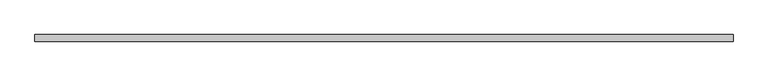
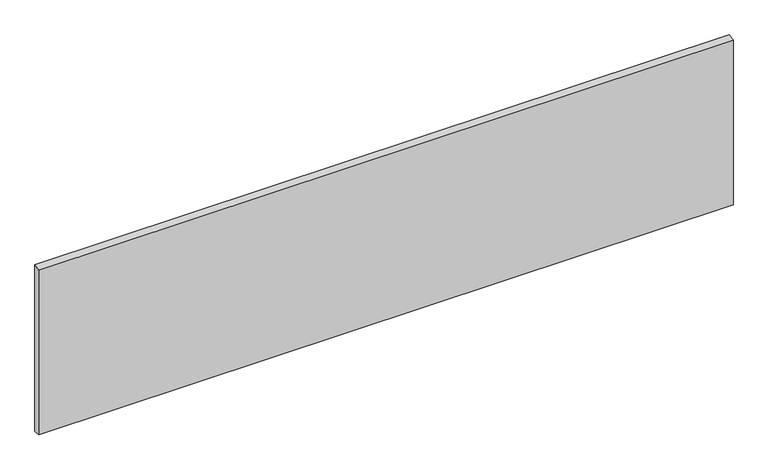
"""IFC4 building model written with IfcOpenShell, lengths in millimetres: proxy geometry, Plywood018 952 : Plywood018 952."""

from ifc_helpers import new_model, si_unit, frame, origin, place, context, project, spatial, polyline, outline, extrude, source, transform, mapped, element, save


def generic_models_6d488722(model_context):
    return source(origin(), model_context, "Body", "SweptSolid", [
        extrude(outline(polyline([(10417.7250834, 42906.696), (10417.7250834, 43408.1095103), (10436.7750834, 43412.8720103), (10436.7750834, 42906.696), (10417.7250834, 42906.696)])), frame((3694.2883192, 0.0, 0.0), z_axis=(1.0, 0.0, 0.0), x_axis=(0.0, 1.0, 0.0)), (0.0, 0.0, 1.0), 2000.0),
    ])


if __name__ == "__main__":
    model = new_model("IFC4")
    model_context = context("Model", 3, world=origin())
    ifc_project = project(units=[si_unit("LENGTHUNIT", "METRE", prefix="MILLI")], contexts=[model_context])
    site = spatial("IfcSite", under=ifc_project)
    building = spatial("IfcBuilding", under=site)
    placement = place(None, origin())
    generic_models_shape = generic_models_6d488722(model_context)
    element("IfcBuildingElementProxy", 1, Name="Plywood018 952 : Plywood018 952", ObjectType="Plywood018 952 : Plywood018 952", at=placement, inside=building, context=model_context, shape_type="MappedRepresentation", body=[
        mapped(generic_models_shape, transform((0.0, 0.0, 0.0), x_axis=(1.0, 0.0, 0.0), y_axis=(0.0, 1.0, 0.0), z_axis=(0.0, 0.0, 1.0))),
    ])
    save(model, "model.ifc")

# Revit data of these elements
# Type "Plywood018 952 : Plywood018 952"
#   NameOverride = "Plywood018"
# Element 1 (IfcBuildingElementProxy, "Plywood018 952 : Plywood018 952")
#   Materials on its faces: "CDX PLYWOOD - SEE STRUCTURAL DWGS"
# Materials
#   "CDX PLYWOOD - SEE STRUCTURAL DWGS": class "Unassigned", colour RGB 177 130 114, transparency 0, Cost = 0
